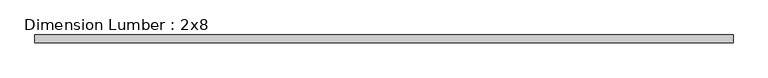
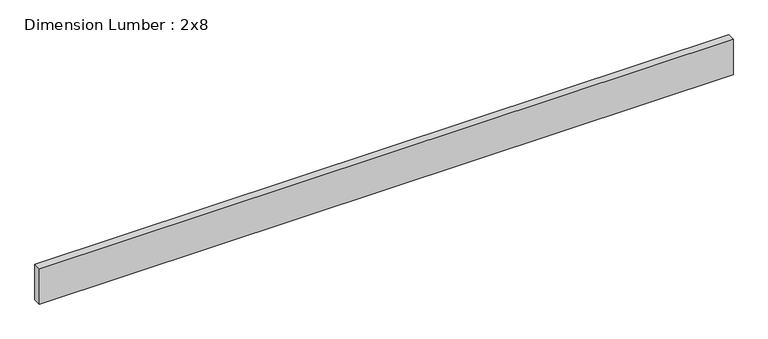
"""IFC4 building model written with IfcOpenShell, lengths in millimetres: beam geometry, Dimension Lumber : 2x8."""

import ifcopenshell
import ifcopenshell.guid

model = None  # the IFC model being written
_history = None  # IfcOwnerHistory: only IFC2X3 demands one
_inside = {}  # id of a spatial element -> (the spatial element, [elements in it])
_under = {}  # id of a project, library or spatial element -> (it, [spatial elements below it])
_declared = {}  # id of a project -> (the project, [libraries it declares])
_typed = {}  # id of a type object -> (the type object, [elements of that type])
_made_of = {}  # id of a material, layer set ... -> (it, [elements and type objects made of it])


def new_model(schema):
    """Start an empty IFC model of exactly this schema.

    Asked for "IFC4X3", IfcOpenShell would pick the latest addendum, in which some entities
    have other attributes; the version numbers below select the first issue.
    IFC2X3 requires an IfcOwnerHistory on every rooted entity: one is made here for all.
    """
    global model, _history
    if schema == "IFC4X3":
        model = ifcopenshell.file(schema_version=(4, 3, 0, 0))
    else:
        model = ifcopenshell.file(schema=schema)
    _inside.clear()
    _under.clear()
    _declared.clear()
    _typed.clear()
    _made_of.clear()
    _history = None
    if model.schema == "IFC2X3":
        org = make("IfcOrganization", Name="unknown")
        user = make(
            "IfcPersonAndOrganization",
            ThePerson=make("IfcPerson", FamilyName="unknown"),
            TheOrganization=org,
        )
        app = make(
            "IfcApplication",
            ApplicationDeveloper=org,
            Version="unknown",
            ApplicationFullName="unknown",
            ApplicationIdentifier="unknown",
        )
        _history = make(
            "IfcOwnerHistory",
            OwningUser=user,
            OwningApplication=app,
            ChangeAction="ADDED",
            CreationDate=0,
        )
    return model


def make(cls, **values):
    """One entity of the class cls with the attributes given. An attribute that is None is left unset."""
    return model.create_entity(
        cls, **{name: value for name, value in values.items() if value is not None}
    )


def rooted(cls, **values):
    """An entity with a GlobalId (a new one), such as an element, a storey or a relation."""
    return make(cls, GlobalId=ifcopenshell.guid.new(), OwnerHistory=_history, **values)


def si_unit(unit_type, name, prefix=None):
    """IfcSIUnit, for example si_unit("LENGTHUNIT", "METRE", prefix="MILLI")."""
    return make("IfcSIUnit", UnitType=unit_type, Prefix=prefix, Name=name)


def assignment(units):
    """IfcUnitAssignment: the units of a project."""
    return None if units is None else make("IfcUnitAssignment", Units=units)


def point(xyz):
    """IfcCartesianPoint."""
    return None if xyz is None else make("IfcCartesianPoint", Coordinates=xyz)


def direction(xyz):
    """IfcDirection."""
    return None if xyz is None else make("IfcDirection", DirectionRatios=xyz)


def frame(location, z_axis=None, x_axis=None):
    """IfcAxis2Placement3D, a coordinate frame: its origin and axes. An axis left out is left unset."""
    return make(
        "IfcAxis2Placement3D",
        Location=point(location),
        Axis=direction(z_axis),
        RefDirection=direction(x_axis),
    )


def origin():
    """The frame at (0, 0, 0) with its axes left unset."""
    return frame((0.0, 0.0, 0.0))


def place(relative_to, where):
    """IfcLocalPlacement: puts the frame where relative to a parent placement (None: the world)."""
    return make(
        "IfcLocalPlacement", PlacementRelTo=relative_to, RelativePlacement=where
    )


def context(
    kind, dimensions, precision=None, world=None, true_north=None, identifier=None
):
    """IfcGeometricRepresentationContext, for example the 3D "Model" context."""
    return make(
        "IfcGeometricRepresentationContext",
        ContextIdentifier=identifier,
        ContextType=kind,
        CoordinateSpaceDimension=dimensions,
        Precision=precision,
        WorldCoordinateSystem=world,
        TrueNorth=true_north,
    )


def project(units=None, contexts=None):
    """IfcProject with its units and contexts."""
    return rooted(
        "IfcProject",
        Name="project",
        RepresentationContexts=contexts,
        UnitsInContext=assignment(units),
    )


def spatial(cls, under=None, at=None, **own):
    """A site, building, storey or space (cls), placed at a placement, below another one or the project."""
    s = rooted(cls, ObjectPlacement=at, **own)
    if under is not None:
        _under.setdefault(under.id(), (under, []))[1].append(s)
    return s


def polyline(points):
    """IfcPolyline through the points."""
    return make("IfcPolyline", Points=[point(p) for p in points])


def outline(outer, holes=None, kind="AREA"):
    """IfcArbitraryClosedProfileDef: a profile drawn as a closed curve; with holes, ...WithVoids."""
    if holes is None:
        return make("IfcArbitraryClosedProfileDef", ProfileType=kind, OuterCurve=outer)
    return make(
        "IfcArbitraryProfileDefWithVoids",
        ProfileType=kind,
        OuterCurve=outer,
        InnerCurves=holes,
    )


def extrude(swept, where, along, depth):
    """IfcExtrudedAreaSolid: the profile swept, set in the frame where, extruded along a direction by depth."""
    return make(
        "IfcExtrudedAreaSolid",
        SweptArea=swept,
        Position=where,
        ExtrudedDirection=direction(along),
        Depth=depth,
    )


def shape(context_of_items, identifier, shape_type, items):
    """IfcShapeRepresentation: the items that make up one representation, for example the "Body"."""
    return make(
        "IfcShapeRepresentation",
        ContextOfItems=context_of_items,
        RepresentationIdentifier=identifier,
        RepresentationType=shape_type,
        Items=items,
    )


def source(mapping_origin, context_of_items, identifier, shape_type, items):
    """IfcRepresentationMap: a shape defined once, which mapped items show again and again."""
    return make(
        "IfcRepresentationMap",
        MappingOrigin=mapping_origin,
        MappedRepresentation=shape(context_of_items, identifier, shape_type, items),
    )


def transform(
    local_origin,
    x_axis=None,
    y_axis=None,
    z_axis=None,
    scale=None,
    scale2=None,
    scale3=None,
    uniform=True,
):
    """IfcCartesianTransformationOperator3D, or its non-uniform kind. x_axis, y_axis, z_axis: its Axis1, 2, 3."""
    if uniform:
        return make(
            "IfcCartesianTransformationOperator3D",
            Axis1=direction(x_axis),
            Axis2=direction(y_axis),
            LocalOrigin=point(local_origin),
            Scale=scale,
            Axis3=direction(z_axis),
        )
    return make(
        "IfcCartesianTransformationOperator3DnonUniform",
        Axis1=direction(x_axis),
        Axis2=direction(y_axis),
        LocalOrigin=point(local_origin),
        Scale=scale,
        Axis3=direction(z_axis),
        Scale2=scale2,
        Scale3=scale3,
    )


def mapped(mapping_source, mapping_target):
    """IfcMappedItem: shows the shape of a source again, moved by a transform."""
    return make(
        "IfcMappedItem", MappingSource=mapping_source, MappingTarget=mapping_target
    )


def made_of(thing, what):
    """Note that an element or type object is made of a material, layer set ...; save() writes the relation."""
    if what is not None:
        _made_of.setdefault(what.id(), (what, []))[1].append(thing)
    return thing


def element(
    cls,
    number,
    at=None,
    inside=None,
    cuts=None,
    type_object=None,
    material=None,
    context=None,
    identifier="Body",
    shape_type=None,
    held_by="IfcProductDefinitionShape",
    body=None,
    shapes=None,
    **own,
):
    """One element of the class cls, such as IfcWall. Its Tag is "e" and its number.

    at: its placement. inside: the storey or other place that contains it. cuts: it is an
    opening in that element (IfcRelVoidsElement). A single representation is given by context,
    identifier, shape_type and body (its items); several are given by shapes. held_by: the class
    of the entity that holds the representations. save() writes the other relations.
    """
    e = rooted(cls, Tag="e%d" % number, ObjectPlacement=at, **own)
    if body is not None:
        shapes = [shape(context, identifier, shape_type, body)]
    if shapes is not None:
        e.Representation = make(held_by, Representations=shapes)
    if inside is not None:
        _inside.setdefault(inside.id(), (inside, []))[1].append(e)
    if cuts is not None:
        rooted(
            "IfcRelVoidsElement", RelatingBuildingElement=cuts, RelatedOpeningElement=e
        )
    if type_object is not None:
        _typed.setdefault(type_object.id(), (type_object, []))[1].append(e)
    return made_of(e, material)


def aggregate(whole, parts):
    """IfcRelAggregates: a whole, such as a stair, and the parts it consists of."""
    return rooted("IfcRelAggregates", RelatingObject=whole, RelatedObjects=parts)


def save(model, path):
    """Write the relations noted so far, then the file.

    IfcRelAggregates (storeys below a building ...), IfcRelContainedInSpatialStructure (elements
    in a storey), IfcRelDefinesByType, IfcRelAssociatesMaterial and IfcRelDeclares: one each for
    every whole, place, type object, material and project.
    """
    for whole, parts in _under.values():
        aggregate(whole, parts)
    for where, things in _inside.values():
        rooted(
            "IfcRelContainedInSpatialStructure",
            RelatedElements=things,
            RelatingStructure=where,
        )
    for kind, things in _typed.values():
        rooted("IfcRelDefinesByType", RelatedObjects=things, RelatingType=kind)
    for what, things in _made_of.values():
        rooted("IfcRelAssociatesMaterial", RelatedObjects=things, RelatingMaterial=what)
    for by, libraries in _declared.values():
        rooted("IfcRelDeclares", RelatingContext=by, RelatedDefinitions=libraries)
    model.write(path)


def dimension_lumber_2x8_9f3a7dbc(model_context):
    return source(origin(), model_context, "Body", "SweptSolid", [
        extrude(outline(polyline([(2227.6894756, -19.05), (-1175.9105244, -19.05), (-1175.9105244, 19.05), (2227.6894756, 19.05), (2227.6894756, -19.05)])), frame((0.0, 0.0, -92.075), z_axis=(0.0, 0.0, 1.0), x_axis=(1.0, 0.0, 0.0)), (0.0, 0.0, 1.0), 184.15),
    ])


if __name__ == "__main__":
    model = new_model("IFC4")
    model_context = context("Model", 3, world=origin())
    ifc_project = project(units=[si_unit("LENGTHUNIT", "METRE", prefix="MILLI")], contexts=[model_context])
    site = spatial("IfcSite", under=ifc_project)
    building = spatial("IfcBuilding", under=site)
    placement = place(None, origin())
    dimension_lumber_2x8_shape = dimension_lumber_2x8_9f3a7dbc(model_context)
    element("IfcBeam", 1, ObjectType="Dimension Lumber : 2x8", at=placement, inside=building, context=model_context, shape_type="MappedRepresentation", body=[
        mapped(dimension_lumber_2x8_shape, transform((0.0, 0.0, 0.0), x_axis=(1.0, 0.0, 0.0), y_axis=(0.0, 1.0, 0.0), z_axis=(0.0, 0.0, 1.0))),
    ])
    save(model, "model.ifc")

# Revit data of these elements
# Type "Dimension Lumber : 2x8"
#   Assembly Code = "B10"
#   A = 0.0755556 SF
#   Length [instance default] = 5' - 0"
#   b = 0' - 1 1/2"
#   d = 0' - 7 1/4"
#   Structural Material [instance default] = PRE-ENGINEERED TRUSS @ 24" O.C.
# Element 1 (IfcBeam, "Dimension Lumber : 2x8")
#   Structural Material = 2 X 8 FIELD FRAMED PURLINS
#   Materials on its faces: "2 X 8 FIELD FRAMED PURLINS"
# Materials
#   "PRE-ENGINEERED TRUSS @ 24\" O.C.": class "Wood", colour RGB 255 255 255, transparency 0, Description = "Pinus Echinata", Cost = 0
#   "2 X 8 FIELD FRAMED PURLINS": class "Wood", colour RGB 234 198 147, transparency 0, Description = "Pinus Echinata", Cost = 0
